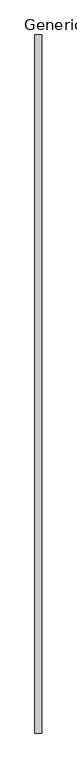
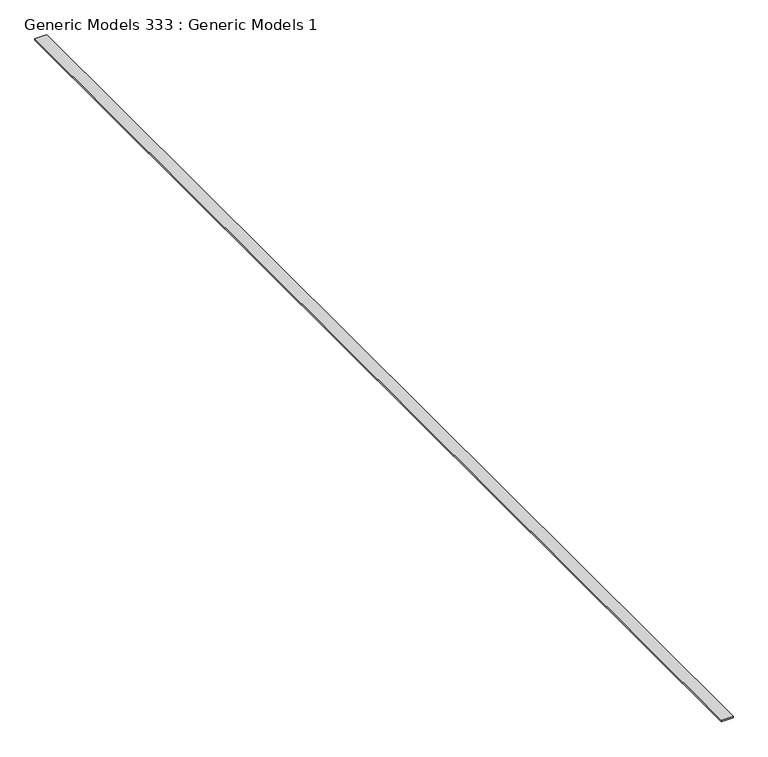
"""IFC4 building model written with IfcOpenShell, lengths in millimetres: proxy geometry, Generic Models 333 : Generic Models 1."""

from ifc_helpers import new_model, si_unit, frame, origin, place, context, project, spatial, polyline, outline, extrude, source, transform, mapped, element, save


def generic_models_333_generic_models_1_0a9324d4(model_context):
    return source(origin(), model_context, "Body", "SweptSolid", [
        extrude(outline(polyline([(0.0, -76.2), (0.0, 0.0), (7620.0, 0.0), (7620.0, -76.2), (0.0, -76.2)])), frame((8421.9756095, 551.8769662, 126108.2398165), z_axis=(1.2555512185485895e-12, 0.0, 1.0), x_axis=(0.0, -1.0, 0.0)), (0.0, 0.0, 1.0), 11.1125),
    ])


if __name__ == "__main__":
    model = new_model("IFC4")
    model_context = context("Model", 3, world=origin())
    ifc_project = project(units=[si_unit("LENGTHUNIT", "METRE", prefix="MILLI")], contexts=[model_context])
    site = spatial("IfcSite", under=ifc_project)
    building = spatial("IfcBuilding", under=site)
    placement = place(None, origin())
    generic_models_333_generic_models_1_shape = generic_models_333_generic_models_1_0a9324d4(model_context)
    element("IfcBuildingElementProxy", 1, Name="Generic Models 333 : Generic Models 1", ObjectType="Generic Models 333 : Generic Models 1", at=placement, inside=building, context=model_context, shape_type="MappedRepresentation", body=[
        mapped(generic_models_333_generic_models_1_shape, transform((0.0, 0.0, 0.0), x_axis=(1.0, 0.0, 0.0), y_axis=(0.0, 1.0, 0.0), z_axis=(0.0, 0.0, 1.0))),
    ])
    save(model, "model.ifc")

# Revit data of these elements
# Element 1 (IfcBuildingElementProxy, "Generic Models 333 : Generic Models 1")
#   Materials on its faces: "_SIDING VENT - COR-A-VENT - 7/16\" X 3\""
# Materials
#   "_SIDING VENT - COR-A-VENT - 7/16\" X 3\"": class "Generic", colour RGB 190 220 196, transparency 0, Cost = 0
